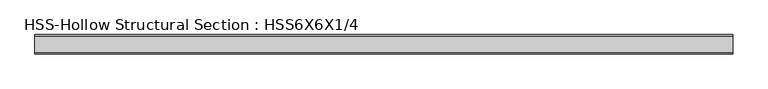
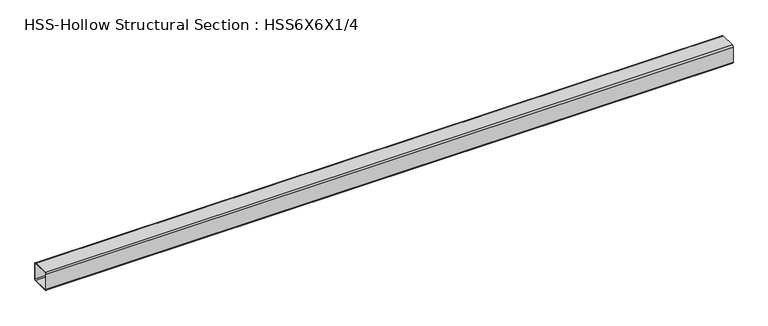
"""IFC4 building model written with IfcOpenShell, lengths in millimetres: beam geometry, HSS-Hollow Structural Section : HSS6X6X1/4."""

import ifcopenshell
import ifcopenshell.guid

model = None  # the IFC model being written
_history = None  # IfcOwnerHistory: only IFC2X3 demands one
_inside = {}  # id of a spatial element -> (the spatial element, [elements in it])
_under = {}  # id of a project, library or spatial element -> (it, [spatial elements below it])
_declared = {}  # id of a project -> (the project, [libraries it declares])
_typed = {}  # id of a type object -> (the type object, [elements of that type])
_made_of = {}  # id of a material, layer set ... -> (it, [elements and type objects made of it])


def new_model(schema):
    """Start an empty IFC model of exactly this schema.

    Asked for "IFC4X3", IfcOpenShell would pick the latest addendum, in which some entities
    have other attributes; the version numbers below select the first issue.
    IFC2X3 requires an IfcOwnerHistory on every rooted entity: one is made here for all.
    """
    global model, _history
    if schema == "IFC4X3":
        model = ifcopenshell.file(schema_version=(4, 3, 0, 0))
    else:
        model = ifcopenshell.file(schema=schema)
    _inside.clear()
    _under.clear()
    _declared.clear()
    _typed.clear()
    _made_of.clear()
    _history = None
    if model.schema == "IFC2X3":
        org = make("IfcOrganization", Name="unknown")
        user = make(
            "IfcPersonAndOrganization",
            ThePerson=make("IfcPerson", FamilyName="unknown"),
            TheOrganization=org,
        )
        app = make(
            "IfcApplication",
            ApplicationDeveloper=org,
            Version="unknown",
            ApplicationFullName="unknown",
            ApplicationIdentifier="unknown",
        )
        _history = make(
            "IfcOwnerHistory",
            OwningUser=user,
            OwningApplication=app,
            ChangeAction="ADDED",
            CreationDate=0,
        )
    return model


def make(cls, **values):
    """One entity of the class cls with the attributes given. An attribute that is None is left unset."""
    return model.create_entity(
        cls, **{name: value for name, value in values.items() if value is not None}
    )


def rooted(cls, **values):
    """An entity with a GlobalId (a new one), such as an element, a storey or a relation."""
    return make(cls, GlobalId=ifcopenshell.guid.new(), OwnerHistory=_history, **values)


def si_unit(unit_type, name, prefix=None):
    """IfcSIUnit, for example si_unit("LENGTHUNIT", "METRE", prefix="MILLI")."""
    return make("IfcSIUnit", UnitType=unit_type, Prefix=prefix, Name=name)


def assignment(units):
    """IfcUnitAssignment: the units of a project."""
    return None if units is None else make("IfcUnitAssignment", Units=units)


def point(xyz):
    """IfcCartesianPoint."""
    return None if xyz is None else make("IfcCartesianPoint", Coordinates=xyz)


def direction(xyz):
    """IfcDirection."""
    return None if xyz is None else make("IfcDirection", DirectionRatios=xyz)


def frame(location, z_axis=None, x_axis=None):
    """IfcAxis2Placement3D, a coordinate frame: its origin and axes. An axis left out is left unset."""
    return make(
        "IfcAxis2Placement3D",
        Location=point(location),
        Axis=direction(z_axis),
        RefDirection=direction(x_axis),
    )


def frame_2d(location, x_axis=None):
    """IfcAxis2Placement2D, a coordinate frame in the plane: its origin and x axis."""
    return make(
        "IfcAxis2Placement2D", Location=point(location), RefDirection=direction(x_axis)
    )


def origin():
    """The frame at (0, 0, 0) with its axes left unset."""
    return frame((0.0, 0.0, 0.0))


def place(relative_to, where):
    """IfcLocalPlacement: puts the frame where relative to a parent placement (None: the world)."""
    return make(
        "IfcLocalPlacement", PlacementRelTo=relative_to, RelativePlacement=where
    )


def context(
    kind, dimensions, precision=None, world=None, true_north=None, identifier=None
):
    """IfcGeometricRepresentationContext, for example the 3D "Model" context."""
    return make(
        "IfcGeometricRepresentationContext",
        ContextIdentifier=identifier,
        ContextType=kind,
        CoordinateSpaceDimension=dimensions,
        Precision=precision,
        WorldCoordinateSystem=world,
        TrueNorth=true_north,
    )


def project(units=None, contexts=None):
    """IfcProject with its units and contexts."""
    return rooted(
        "IfcProject",
        Name="project",
        RepresentationContexts=contexts,
        UnitsInContext=assignment(units),
    )


def spatial(cls, under=None, at=None, **own):
    """A site, building, storey or space (cls), placed at a placement, below another one or the project."""
    s = rooted(cls, ObjectPlacement=at, **own)
    if under is not None:
        _under.setdefault(under.id(), (under, []))[1].append(s)
    return s


def polyline(points):
    """IfcPolyline through the points."""
    return make("IfcPolyline", Points=[point(p) for p in points])


def circle_curve(where, radius):
    """IfcCircle in the frame where."""
    return make("IfcCircle", Position=where, Radius=radius)


def trimmed(basis, trim1, trim2, sense, master):
    """IfcTrimmedCurve: the piece of a basis curve between two trims."""
    return make(
        "IfcTrimmedCurve",
        BasisCurve=basis,
        Trim1=trim1,
        Trim2=trim2,
        SenseAgreement=sense,
        MasterRepresentation=master,
    )


def segment(curve, same_sense, transition):
    """IfcCompositeCurveSegment."""
    return make(
        "IfcCompositeCurveSegment",
        Transition=transition,
        SameSense=same_sense,
        ParentCurve=curve,
    )


def composite_curve(segments, self_intersect=None):
    """IfcCompositeCurve: segments joined end to end."""
    return make("IfcCompositeCurve", Segments=segments, SelfIntersect=self_intersect)


def outline(outer, holes=None, kind="AREA"):
    """IfcArbitraryClosedProfileDef: a profile drawn as a closed curve; with holes, ...WithVoids."""
    if holes is None:
        return make("IfcArbitraryClosedProfileDef", ProfileType=kind, OuterCurve=outer)
    return make(
        "IfcArbitraryProfileDefWithVoids",
        ProfileType=kind,
        OuterCurve=outer,
        InnerCurves=holes,
    )


def extrude(swept, where, along, depth):
    """IfcExtrudedAreaSolid: the profile swept, set in the frame where, extruded along a direction by depth."""
    return make(
        "IfcExtrudedAreaSolid",
        SweptArea=swept,
        Position=where,
        ExtrudedDirection=direction(along),
        Depth=depth,
    )


def shape(context_of_items, identifier, shape_type, items):
    """IfcShapeRepresentation: the items that make up one representation, for example the "Body"."""
    return make(
        "IfcShapeRepresentation",
        ContextOfItems=context_of_items,
        RepresentationIdentifier=identifier,
        RepresentationType=shape_type,
        Items=items,
    )


def source(mapping_origin, context_of_items, identifier, shape_type, items):
    """IfcRepresentationMap: a shape defined once, which mapped items show again and again."""
    return make(
        "IfcRepresentationMap",
        MappingOrigin=mapping_origin,
        MappedRepresentation=shape(context_of_items, identifier, shape_type, items),
    )


def transform(
    local_origin,
    x_axis=None,
    y_axis=None,
    z_axis=None,
    scale=None,
    scale2=None,
    scale3=None,
    uniform=True,
):
    """IfcCartesianTransformationOperator3D, or its non-uniform kind. x_axis, y_axis, z_axis: its Axis1, 2, 3."""
    if uniform:
        return make(
            "IfcCartesianTransformationOperator3D",
            Axis1=direction(x_axis),
            Axis2=direction(y_axis),
            LocalOrigin=point(local_origin),
            Scale=scale,
            Axis3=direction(z_axis),
        )
    return make(
        "IfcCartesianTransformationOperator3DnonUniform",
        Axis1=direction(x_axis),
        Axis2=direction(y_axis),
        LocalOrigin=point(local_origin),
        Scale=scale,
        Axis3=direction(z_axis),
        Scale2=scale2,
        Scale3=scale3,
    )


def mapped(mapping_source, mapping_target):
    """IfcMappedItem: shows the shape of a source again, moved by a transform."""
    return make(
        "IfcMappedItem", MappingSource=mapping_source, MappingTarget=mapping_target
    )


def made_of(thing, what):
    """Note that an element or type object is made of a material, layer set ...; save() writes the relation."""
    if what is not None:
        _made_of.setdefault(what.id(), (what, []))[1].append(thing)
    return thing


def element(
    cls,
    number,
    at=None,
    inside=None,
    cuts=None,
    type_object=None,
    material=None,
    context=None,
    identifier="Body",
    shape_type=None,
    held_by="IfcProductDefinitionShape",
    body=None,
    shapes=None,
    **own,
):
    """One element of the class cls, such as IfcWall. Its Tag is "e" and its number.

    at: its placement. inside: the storey or other place that contains it. cuts: it is an
    opening in that element (IfcRelVoidsElement). A single representation is given by context,
    identifier, shape_type and body (its items); several are given by shapes. held_by: the class
    of the entity that holds the representations. save() writes the other relations.
    """
    e = rooted(cls, Tag="e%d" % number, ObjectPlacement=at, **own)
    if body is not None:
        shapes = [shape(context, identifier, shape_type, body)]
    if shapes is not None:
        e.Representation = make(held_by, Representations=shapes)
    if inside is not None:
        _inside.setdefault(inside.id(), (inside, []))[1].append(e)
    if cuts is not None:
        rooted(
            "IfcRelVoidsElement", RelatingBuildingElement=cuts, RelatedOpeningElement=e
        )
    if type_object is not None:
        _typed.setdefault(type_object.id(), (type_object, []))[1].append(e)
    return made_of(e, material)


def aggregate(whole, parts):
    """IfcRelAggregates: a whole, such as a stair, and the parts it consists of."""
    return rooted("IfcRelAggregates", RelatingObject=whole, RelatedObjects=parts)


def save(model, path):
    """Write the relations noted so far, then the file.

    IfcRelAggregates (storeys below a building ...), IfcRelContainedInSpatialStructure (elements
    in a storey), IfcRelDefinesByType, IfcRelAssociatesMaterial and IfcRelDeclares: one each for
    every whole, place, type object, material and project.
    """
    for whole, parts in _under.values():
        aggregate(whole, parts)
    for where, things in _inside.values():
        rooted(
            "IfcRelContainedInSpatialStructure",
            RelatedElements=things,
            RelatingStructure=where,
        )
    for kind, things in _typed.values():
        rooted("IfcRelDefinesByType", RelatedObjects=things, RelatingType=kind)
    for what, things in _made_of.values():
        rooted("IfcRelAssociatesMaterial", RelatedObjects=things, RelatingMaterial=what)
    for by, libraries in _declared.values():
        rooted("IfcRelDeclares", RelatingContext=by, RelatedDefinitions=libraries)
    model.write(path)


def hss_hollow_structural_section_hss6x6x1_4_db1f6c85(model_context):
    return source(origin(), model_context, "Body", "SweptSolid", [
        extrude(outline(composite_curve([segment(polyline([(76.2, 64.3636), (76.2, -64.3636)]), True, "CONTINUOUS"), segment(trimmed(circle_curve(frame_2d((64.3636, -64.3636)), 11.8364), [point((76.2, -64.3636))], [point((64.3636, -76.2))], False, "CARTESIAN"), True, "CONTINUOUS"), segment(polyline([(64.3636, -76.2), (-64.3636, -76.2)]), True, "CONTINUOUS"), segment(trimmed(circle_curve(frame_2d((-64.3636, -64.3636)), 11.8364), [point((-64.3636, -76.2))], [point((-76.2, -64.3636))], False, "CARTESIAN"), True, "CONTINUOUS"), segment(polyline([(-76.2, -64.3636), (-76.2, 64.3636)]), True, "CONTINUOUS"), segment(trimmed(circle_curve(frame_2d((-64.3636, 64.3636)), 11.8364), [point((-76.2, 64.3636))], [point((-64.3636, 76.2))], False, "CARTESIAN"), True, "CONTINUOUS"), segment(polyline([(-64.3636, 76.2), (64.3636, 76.2)]), True, "CONTINUOUS"), segment(trimmed(circle_curve(frame_2d((64.3636, 64.3636)), 11.8364), [point((64.3636, 76.2))], [point((76.2, 64.3636))], False, "CARTESIAN"), True, "CONTINUOUS")], self_intersect=False), holes=[composite_curve([segment(trimmed(circle_curve(frame_2d((-64.3636, 64.3636)), 5.9182), [point((-64.3636, 70.2818))], [point((-70.2818, 64.3636))], True, "CARTESIAN"), True, "CONTINUOUS"), segment(polyline([(-70.2818, 64.3636), (-70.2818, -64.3636)]), True, "CONTINUOUS"), segment(trimmed(circle_curve(frame_2d((-64.3636, -64.3636)), 5.9182), [point((-70.2818, -64.3636))], [point((-64.3636, -70.2818))], True, "CARTESIAN"), True, "CONTINUOUS"), segment(polyline([(-64.3636, -70.2818), (64.3636, -70.2818)]), True, "CONTINUOUS"), segment(trimmed(circle_curve(frame_2d((64.3636, -64.3636)), 5.9182), [point((64.3636, -70.2818))], [point((70.2818, -64.3636))], True, "CARTESIAN"), True, "CONTINUOUS"), segment(polyline([(70.2818, -64.3636), (70.2818, 64.3636)]), True, "CONTINUOUS"), segment(trimmed(circle_curve(frame_2d((64.3636, 64.3636)), 5.9182), [point((70.2818, 64.3636))], [point((64.3636, 70.2818))], True, "CARTESIAN"), True, "CONTINUOUS"), segment(polyline([(64.3636, 70.2818), (-64.3636, 70.2818)]), True, "CONTINUOUS")], self_intersect=False)]), frame((-2751.9238693, 0.0, 0.0), z_axis=(1.0, 0.0, 0.0), x_axis=(0.0, 1.0, 0.0)), (0.0, 0.0, 1.0), 5507.8238693),
    ])


if __name__ == "__main__":
    model = new_model("IFC4")
    model_context = context("Model", 3, world=origin())
    ifc_project = project(units=[si_unit("LENGTHUNIT", "METRE", prefix="MILLI")], contexts=[model_context])
    site = spatial("IfcSite", under=ifc_project)
    building = spatial("IfcBuilding", under=site)
    placement = place(None, origin())
    hss_hollow_structural_section_hss6x6x1_4_shape = hss_hollow_structural_section_hss6x6x1_4_db1f6c85(model_context)
    element("IfcBeam", 1, ObjectType="HSS-Hollow Structural Section : HSS6X6X1/4", at=placement, inside=building, context=model_context, shape_type="MappedRepresentation", body=[
        mapped(hss_hollow_structural_section_hss6x6x1_4_shape, transform((0.0, 0.0, 0.0), x_axis=(1.0, 0.0, 0.0), y_axis=(0.0, 1.0, 0.0), z_axis=(0.0, 0.0, 1.0))),
    ])
    save(model, "model.ifc")

# Revit data of these elements
# Type "HSS-Hollow Structural Section : HSS6X6X1/4"
#   Assembly Code = "B10"
#   Shape = "Square"
#   W = 19
#   Ht = 0' - 6"
#   Length [instance default] = 5' - 0"
#   b = 0' - 6"
#   kr = 0' - 0.466"
#   t = 0' - 0.233"
#   A = 0.0363889 SF
#   Structural Material [instance default] = Steel ASTM A500, Grade B, Rectangular and Square
# Element 1 (IfcBeam, "HSS-Hollow Structural Section : HSS6X6X1/4")
#   Materials on its faces: "Steel ASTM A500, Grade B, Rectangular and Square"
# Materials
#   "Steel ASTM A500, Grade B, Rectangular and Square": class "Metal", colour RGB 199 199 199, transparency 0, Description = "Carbon steel", Cost = 0
